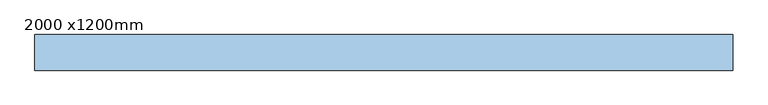
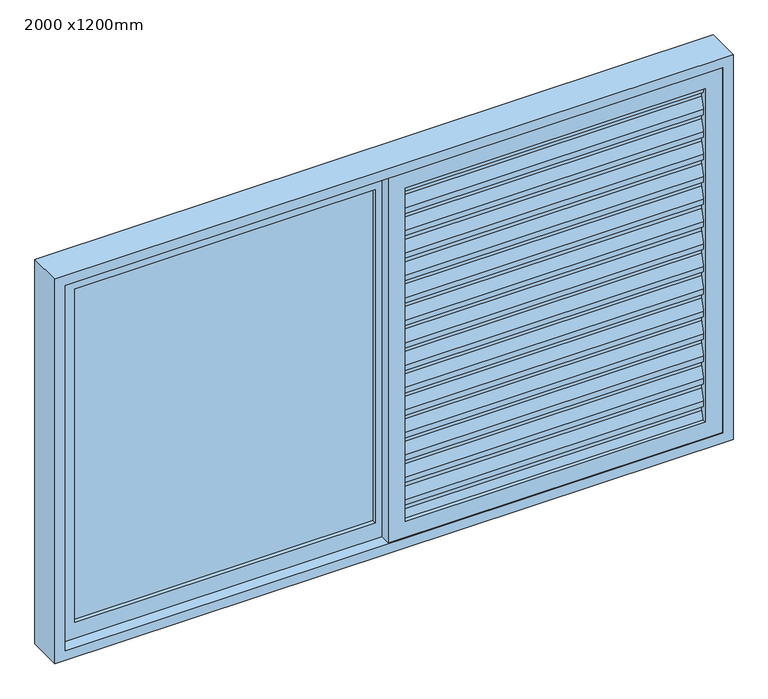
"""IFC4 building model written with IfcOpenShell, lengths in millimetres: window geometry, Janela Veneziana de Correr - 3 Folhas : 2000 x1200mm."""

import ifcopenshell
import ifcopenshell.guid

model = None  # the IFC model being written
_history = None  # IfcOwnerHistory: only IFC2X3 demands one
_inside = {}  # id of a spatial element -> (the spatial element, [elements in it])
_under = {}  # id of a project, library or spatial element -> (it, [spatial elements below it])
_declared = {}  # id of a project -> (the project, [libraries it declares])
_typed = {}  # id of a type object -> (the type object, [elements of that type])
_made_of = {}  # id of a material, layer set ... -> (it, [elements and type objects made of it])


def new_model(schema):
    """Start an empty IFC model of exactly this schema.

    Asked for "IFC4X3", IfcOpenShell would pick the latest addendum, in which some entities
    have other attributes; the version numbers below select the first issue.
    IFC2X3 requires an IfcOwnerHistory on every rooted entity: one is made here for all.
    """
    global model, _history
    if schema == "IFC4X3":
        model = ifcopenshell.file(schema_version=(4, 3, 0, 0))
    else:
        model = ifcopenshell.file(schema=schema)
    _inside.clear()
    _under.clear()
    _declared.clear()
    _typed.clear()
    _made_of.clear()
    _history = None
    if model.schema == "IFC2X3":
        org = make("IfcOrganization", Name="unknown")
        user = make(
            "IfcPersonAndOrganization",
            ThePerson=make("IfcPerson", FamilyName="unknown"),
            TheOrganization=org,
        )
        app = make(
            "IfcApplication",
            ApplicationDeveloper=org,
            Version="unknown",
            ApplicationFullName="unknown",
            ApplicationIdentifier="unknown",
        )
        _history = make(
            "IfcOwnerHistory",
            OwningUser=user,
            OwningApplication=app,
            ChangeAction="ADDED",
            CreationDate=0,
        )
    return model


def make(cls, **values):
    """One entity of the class cls with the attributes given. An attribute that is None is left unset."""
    return model.create_entity(
        cls, **{name: value for name, value in values.items() if value is not None}
    )


def rooted(cls, **values):
    """An entity with a GlobalId (a new one), such as an element, a storey or a relation."""
    return make(cls, GlobalId=ifcopenshell.guid.new(), OwnerHistory=_history, **values)


def si_unit(unit_type, name, prefix=None):
    """IfcSIUnit, for example si_unit("LENGTHUNIT", "METRE", prefix="MILLI")."""
    return make("IfcSIUnit", UnitType=unit_type, Prefix=prefix, Name=name)


def assignment(units):
    """IfcUnitAssignment: the units of a project."""
    return None if units is None else make("IfcUnitAssignment", Units=units)


def point(xyz):
    """IfcCartesianPoint."""
    return None if xyz is None else make("IfcCartesianPoint", Coordinates=xyz)


def direction(xyz):
    """IfcDirection."""
    return None if xyz is None else make("IfcDirection", DirectionRatios=xyz)


def frame(location, z_axis=None, x_axis=None):
    """IfcAxis2Placement3D, a coordinate frame: its origin and axes. An axis left out is left unset."""
    return make(
        "IfcAxis2Placement3D",
        Location=point(location),
        Axis=direction(z_axis),
        RefDirection=direction(x_axis),
    )


def origin():
    """The frame at (0, 0, 0) with its axes left unset."""
    return frame((0.0, 0.0, 0.0))


def place(relative_to, where):
    """IfcLocalPlacement: puts the frame where relative to a parent placement (None: the world)."""
    return make(
        "IfcLocalPlacement", PlacementRelTo=relative_to, RelativePlacement=where
    )


def context(
    kind, dimensions, precision=None, world=None, true_north=None, identifier=None
):
    """IfcGeometricRepresentationContext, for example the 3D "Model" context."""
    return make(
        "IfcGeometricRepresentationContext",
        ContextIdentifier=identifier,
        ContextType=kind,
        CoordinateSpaceDimension=dimensions,
        Precision=precision,
        WorldCoordinateSystem=world,
        TrueNorth=true_north,
    )


def project(units=None, contexts=None):
    """IfcProject with its units and contexts."""
    return rooted(
        "IfcProject",
        Name="project",
        RepresentationContexts=contexts,
        UnitsInContext=assignment(units),
    )


def spatial(cls, under=None, at=None, **own):
    """A site, building, storey or space (cls), placed at a placement, below another one or the project."""
    s = rooted(cls, ObjectPlacement=at, **own)
    if under is not None:
        _under.setdefault(under.id(), (under, []))[1].append(s)
    return s


def polyline(points):
    """IfcPolyline through the points."""
    return make("IfcPolyline", Points=[point(p) for p in points])


def outline(outer, holes=None, kind="AREA"):
    """IfcArbitraryClosedProfileDef: a profile drawn as a closed curve; with holes, ...WithVoids."""
    if holes is None:
        return make("IfcArbitraryClosedProfileDef", ProfileType=kind, OuterCurve=outer)
    return make(
        "IfcArbitraryProfileDefWithVoids",
        ProfileType=kind,
        OuterCurve=outer,
        InnerCurves=holes,
    )


def extrude(swept, where, along, depth):
    """IfcExtrudedAreaSolid: the profile swept, set in the frame where, extruded along a direction by depth."""
    return make(
        "IfcExtrudedAreaSolid",
        SweptArea=swept,
        Position=where,
        ExtrudedDirection=direction(along),
        Depth=depth,
    )


def shape(context_of_items, identifier, shape_type, items):
    """IfcShapeRepresentation: the items that make up one representation, for example the "Body"."""
    return make(
        "IfcShapeRepresentation",
        ContextOfItems=context_of_items,
        RepresentationIdentifier=identifier,
        RepresentationType=shape_type,
        Items=items,
    )


def source(mapping_origin, context_of_items, identifier, shape_type, items):
    """IfcRepresentationMap: a shape defined once, which mapped items show again and again."""
    return make(
        "IfcRepresentationMap",
        MappingOrigin=mapping_origin,
        MappedRepresentation=shape(context_of_items, identifier, shape_type, items),
    )


def transform(
    local_origin,
    x_axis=None,
    y_axis=None,
    z_axis=None,
    scale=None,
    scale2=None,
    scale3=None,
    uniform=True,
):
    """IfcCartesianTransformationOperator3D, or its non-uniform kind. x_axis, y_axis, z_axis: its Axis1, 2, 3."""
    if uniform:
        return make(
            "IfcCartesianTransformationOperator3D",
            Axis1=direction(x_axis),
            Axis2=direction(y_axis),
            LocalOrigin=point(local_origin),
            Scale=scale,
            Axis3=direction(z_axis),
        )
    return make(
        "IfcCartesianTransformationOperator3DnonUniform",
        Axis1=direction(x_axis),
        Axis2=direction(y_axis),
        LocalOrigin=point(local_origin),
        Scale=scale,
        Axis3=direction(z_axis),
        Scale2=scale2,
        Scale3=scale3,
    )


def mapped(mapping_source, mapping_target):
    """IfcMappedItem: shows the shape of a source again, moved by a transform."""
    return make(
        "IfcMappedItem", MappingSource=mapping_source, MappingTarget=mapping_target
    )


def made_of(thing, what):
    """Note that an element or type object is made of a material, layer set ...; save() writes the relation."""
    if what is not None:
        _made_of.setdefault(what.id(), (what, []))[1].append(thing)
    return thing


def element(
    cls,
    number,
    at=None,
    inside=None,
    cuts=None,
    type_object=None,
    material=None,
    context=None,
    identifier="Body",
    shape_type=None,
    held_by="IfcProductDefinitionShape",
    body=None,
    shapes=None,
    **own,
):
    """One element of the class cls, such as IfcWall. Its Tag is "e" and its number.

    at: its placement. inside: the storey or other place that contains it. cuts: it is an
    opening in that element (IfcRelVoidsElement). A single representation is given by context,
    identifier, shape_type and body (its items); several are given by shapes. held_by: the class
    of the entity that holds the representations. save() writes the other relations.
    """
    e = rooted(cls, Tag="e%d" % number, ObjectPlacement=at, **own)
    if body is not None:
        shapes = [shape(context, identifier, shape_type, body)]
    if shapes is not None:
        e.Representation = make(held_by, Representations=shapes)
    if inside is not None:
        _inside.setdefault(inside.id(), (inside, []))[1].append(e)
    if cuts is not None:
        rooted(
            "IfcRelVoidsElement", RelatingBuildingElement=cuts, RelatedOpeningElement=e
        )
    if type_object is not None:
        _typed.setdefault(type_object.id(), (type_object, []))[1].append(e)
    return made_of(e, material)


def aggregate(whole, parts):
    """IfcRelAggregates: a whole, such as a stair, and the parts it consists of."""
    return rooted("IfcRelAggregates", RelatingObject=whole, RelatedObjects=parts)


def save(model, path):
    """Write the relations noted so far, then the file.

    IfcRelAggregates (storeys below a building ...), IfcRelContainedInSpatialStructure (elements
    in a storey), IfcRelDefinesByType, IfcRelAssociatesMaterial and IfcRelDeclares: one each for
    every whole, place, type object, material and project.
    """
    for whole, parts in _under.values():
        aggregate(whole, parts)
    for where, things in _inside.values():
        rooted(
            "IfcRelContainedInSpatialStructure",
            RelatedElements=things,
            RelatingStructure=where,
        )
    for kind, things in _typed.values():
        rooted("IfcRelDefinesByType", RelatedObjects=things, RelatingType=kind)
    for what, things in _made_of.values():
        rooted("IfcRelAssociatesMaterial", RelatedObjects=things, RelatingMaterial=what)
    for by, libraries in _declared.values():
        rooted("IfcRelDeclares", RelatingContext=by, RelatedDefinitions=libraries)
    model.write(path)


def window_2000_x1200mm_dbfbffcb(model_context):
    return source(origin(), model_context, "Body", "SweptSolid", [
        extrude(outline(polyline([(0.6, 1125.0), (0.6, 1105.0), (-6.5028414, 1080.1400549), (-7.5428571, 1080.1400549), (-0.4, 1105.1400549), (-0.4, 1124.0), (-10.4, 1124.0), (-10.4, 1140.1400549), (-0.4, 1175.1400549), (-0.4, 1194.0), (-10.4, 1194.0), (-10.4, 1210.1400549), (-0.4, 1245.1400549), (-0.4, 1264.0), (-10.4, 1264.0), (-10.4, 1280.1400549), (-0.4, 1315.1400549), (-0.4, 1334.0), (-10.4, 1334.0), (-10.4, 1350.1400549), (-0.4, 1385.1400549), (-0.4, 1404.0), (-10.4, 1404.0), (-10.4, 1420.1400549), (-0.4, 1455.1400549), (-0.4, 1474.0), (-10.4, 1474.0), (-10.4, 1490.1400549), (-0.4, 1525.1400549), (-0.4, 1544.0), (-10.4, 1544.0), (-10.4, 1560.1400549), (-0.4, 1595.1400549), (-0.4, 1614.0), (-10.4, 1614.0), (-10.4, 1630.1400549), (-0.4, 1665.1400549), (-0.4, 1684.0), (-10.4, 1684.0), (-10.4, 1700.1400549), (-0.4, 1735.1400549), (-0.4, 1754.0), (-10.4, 1754.0), (-10.4, 1770.1400549), (-0.4, 1805.1400549), (-0.4, 1824.0), (-10.4, 1824.0), (-10.4, 1840.1400549), (-0.4, 1875.1400549), (-0.4, 1894.0), (-10.4, 1894.0), (-10.4, 1910.1400549), (-0.4, 1945.1400549), (-0.4, 1964.0), (-10.4, 1964.0), (-10.4, 1980.1400549), (-0.4, 2015.1400549), (-0.4, 2034.0), (-10.4, 2034.0), (-10.4, 2050.1400549), (-0.4, 2085.1400549), (-0.4, 2104.0), (-10.4, 2104.0), (-10.4, 2120.1400549), (-9.4, 2120.0), (-9.4, 2105.0), (0.6, 2105.0), (0.6, 2085.0), (-9.4, 2050.0), (-9.4, 2035.0), (0.6, 2035.0), (0.6, 2015.0), (-9.4, 1980.0), (-9.4, 1965.0), (0.6, 1965.0), (0.6, 1945.0), (-9.4, 1910.0), (-9.4, 1895.0), (0.6, 1895.0), (0.6, 1875.0), (-9.4, 1840.0), (-9.4, 1825.0), (0.6, 1825.0), (0.6, 1805.0), (-9.4, 1770.0), (-9.4, 1755.0), (0.6, 1755.0), (0.6, 1735.0), (-9.4, 1700.0), (-9.4, 1685.0), (0.6, 1685.0), (0.6, 1665.0), (-9.4, 1630.0), (-9.4, 1615.0), (0.6, 1615.0), (0.6, 1595.0), (-9.4, 1560.0), (-9.4, 1545.0), (0.6, 1545.0), (0.6, 1525.0), (-9.4, 1490.0), (-9.4, 1475.0), (0.6, 1475.0), (0.6, 1455.0), (-9.4, 1420.0), (-9.4, 1405.0), (0.6, 1405.0), (0.6, 1385.0), (-9.4, 1350.0), (-9.4, 1335.0), (0.6, 1335.0), (0.6, 1315.0), (-9.4, 1280.0), (-9.4, 1265.0), (0.6, 1265.0), (0.6, 1245.0), (-9.4, 1210.0), (-9.4, 1195.0), (0.6, 1195.0), (0.6, 1175.0), (-9.4, 1140.0), (-9.4, 1125.0), (0.6, 1125.0)])), frame((35.0, 0.0, 0.0), z_axis=(1.0, 0.0, 0.0), x_axis=(0.0, 1.0, 0.0)), (0.0, 0.0, 1.0), 965.0),
        extrude(outline(polyline([(66.6, 1125.0), (66.6, 1105.0), (59.4971586, 1080.1400549), (58.4571429, 1080.1400549), (65.6, 1105.1400549), (65.6, 1124.0), (55.6, 1124.0), (55.6, 1140.1400549), (65.6, 1175.1400549), (65.6, 1194.0), (55.6, 1194.0), (55.6, 1210.1400549), (65.6, 1245.1400549), (65.6, 1264.0), (55.6, 1264.0), (55.6, 1280.1400549), (65.6, 1315.1400549), (65.6, 1334.0), (55.6, 1334.0), (55.6, 1350.1400549), (65.6, 1385.1400549), (65.6, 1404.0), (55.6, 1404.0), (55.6, 1420.1400549), (65.6, 1455.1400549), (65.6, 1474.0), (55.6, 1474.0), (55.6, 1490.1400549), (65.6, 1525.1400549), (65.6, 1544.0), (55.6, 1544.0), (55.6, 1560.1400549), (65.6, 1595.1400549), (65.6, 1614.0), (55.6, 1614.0), (55.6, 1630.1400549), (65.6, 1665.1400549), (65.6, 1684.0), (55.6, 1684.0), (55.6, 1700.1400549), (65.6, 1735.1400549), (65.6, 1754.0), (55.6, 1754.0), (55.6, 1770.1400549), (65.6, 1805.1400549), (65.6, 1824.0), (55.6, 1824.0), (55.6, 1840.1400549), (65.6, 1875.1400549), (65.6, 1894.0), (55.6, 1894.0), (55.6, 1910.1400549), (65.6, 1945.1400549), (65.6, 1964.0), (55.6, 1964.0), (55.6, 1980.1400549), (65.6, 2015.1400549), (65.6, 2034.0), (55.6, 2034.0), (55.6, 2050.1400549), (65.6, 2085.1400549), (65.6, 2104.0), (55.6, 2104.0), (55.6, 2120.1400549), (56.6, 2120.0), (56.6, 2105.0), (66.6, 2105.0), (66.6, 2085.0), (56.6, 2050.0), (56.6, 2035.0), (66.6, 2035.0), (66.6, 2015.0), (56.6, 1980.0), (56.6, 1965.0), (66.6, 1965.0), (66.6, 1945.0), (56.6, 1910.0), (56.6, 1895.0), (66.6, 1895.0), (66.6, 1875.0), (56.6, 1840.0), (56.6, 1825.0), (66.6, 1825.0), (66.6, 1805.0), (56.6, 1770.0), (56.6, 1755.0), (66.6, 1755.0), (66.6, 1735.0), (56.6, 1700.0), (56.6, 1685.0), (66.6, 1685.0), (66.6, 1665.0), (56.6, 1630.0), (56.6, 1615.0), (66.6, 1615.0), (66.6, 1595.0), (56.6, 1560.0), (56.6, 1545.0), (66.6, 1545.0), (66.6, 1525.0), (56.6, 1490.0), (56.6, 1475.0), (66.6, 1475.0), (66.6, 1455.0), (56.6, 1420.0), (56.6, 1405.0), (66.6, 1405.0), (66.6, 1385.0), (56.6, 1350.0), (56.6, 1335.0), (66.6, 1335.0), (66.6, 1315.0), (56.6, 1280.0), (56.6, 1265.0), (66.6, 1265.0), (66.6, 1245.0), (56.6, 1210.0), (56.6, 1195.0), (66.6, 1195.0), (66.6, 1175.0), (56.6, 1140.0), (56.6, 1125.0), (66.6, 1125.0)])), frame((35.0, 0.0, 0.0), z_axis=(1.0, 0.0, 0.0), x_axis=(0.0, 1.0, 0.0)), (0.0, 0.0, 1.0), 965.0),
        extrude(outline(polyline([(2170.0, -15.0), (1030.0, -15.0), (1030.0, 970.0), (2170.0, 970.0), (2170.0, -15.0)]), holes=[polyline([(2120.0, 35.0), (2120.0, 920.0), (1080.0, 920.0), (1080.0, 35.0), (2120.0, 35.0)])]), frame((0.0, -19.4, 0.0), z_axis=(0.0, 1.0, 0.0), x_axis=(0.0, 0.0, 1.0)), (0.0, 0.0, 1.0), 30.0),
        extrude(outline(polyline([(2170.0, -15.0), (1030.0, -15.0), (1030.0, 970.0), (2170.0, 970.0), (2170.0, -15.0)]), holes=[polyline([(2120.0, 35.0), (2120.0, 920.0), (1080.0, 920.0), (1080.0, 35.0), (2120.0, 35.0)])]), frame((0.0, 46.6, 0.0), z_axis=(0.0, 1.0, 0.0), x_axis=(0.0, 0.0, 1.0)), (0.0, 0.0, 1.0), 30.0),
        extrude(outline(polyline([(-920.0, 25.1), (-920.0, 32.1), (-35.0, 32.1), (-35.0, 25.1), (-920.0, 25.1)])), frame((0.0, 0.0, 1080.0), z_axis=(0.0, 0.0, 1.0), x_axis=(1.0, 0.0, 0.0)), (0.0, 0.0, 1.0), 1040.0),
        extrude(outline(polyline([(2170.0, 15.0), (2170.0, -970.0), (1030.0, -970.0), (1030.0, 15.0), (2170.0, 15.0)]), holes=[polyline([(2120.0, -35.0), (1080.0, -35.0), (1080.0, -920.0), (2120.0, -920.0), (2120.0, -35.0)])]), frame((0.0, 13.6, 0.0), z_axis=(0.0, 1.0, 0.0), x_axis=(0.0, 0.0, 1.0)), (0.0, 0.0, 1.0), 30.0),
        extrude(outline(polyline([(2200.0, 1000.0), (2200.0, -1000.0), (1000.0, -1000.0), (1000.0, 1000.0), (2200.0, 1000.0)]), holes=[polyline([(2170.0, 970.0), (1030.0, 970.0), (1030.0, -970.0), (2170.0, -970.0), (2170.0, 970.0)])]), frame((0.0, -22.4, 0.0), z_axis=(0.0, 1.0, 0.0), x_axis=(0.0, 0.0, 1.0)), (0.0, 0.0, 1.0), 102.0),
    ])


if __name__ == "__main__":
    model = new_model("IFC4")
    model_context = context("Model", 3, world=origin())
    ifc_project = project(units=[si_unit("LENGTHUNIT", "METRE", prefix="MILLI")], contexts=[model_context])
    site = spatial("IfcSite", under=ifc_project)
    building = spatial("IfcBuilding", under=site)
    placement = place(None, origin())
    window_2000_x1200mm_shape = window_2000_x1200mm_dbfbffcb(model_context)
    element("IfcWindow", 1, ObjectType="Janela Veneziana de Correr - 3 Folhas : 2000 x1200mm", at=placement, inside=building, context=model_context, shape_type="MappedRepresentation", body=[
        mapped(window_2000_x1200mm_shape, transform((0.0, 0.0, 0.0), x_axis=(1.0, 0.0, 0.0), y_axis=(0.0, 1.0, 0.0), z_axis=(0.0, 0.0, 1.0))),
    ])
    save(model, "model.ifc")

# Revit data of these elements
# Type "Janela Veneziana de Correr - 3 Folhas : 2000 x1200mm"
#   Type Mark = "J13"
#   SINAPI = ""
#   Tolerância = 0.003 m
#   Módulo Básico M = 0.10 m
#   Largura de Coordenação Modular CM = 2.00 m
#   Largura Vão = 0.965 m
#   Largura Veneziana = 1.00 m
#   Espessura Montante = 0.03 m
#   Largura Batente = 0.10 m
#   L_est_v marco = 0.05 m
#   L_est_h_marco = 0.05 m
#   L_contramarco = 0.03 m
#   Altura de Coordenação Modular CM = 1.20 m
#   Altura Peitoril = 0.95 m
#   Height = 1.20 m
#   Width = 2.00 m
#   Número de Módulos Básicos nM Largura = 20
#   Número de Módulos Básicos nM Altura = 12
#   Material estrutura = Metal - Alumínio
#   Material Quadro = Metal - Alumínio
#   Material Painel = Vidro
#   Type Comments = ""
#   Wall Closure = (empty or 0)
#   Construction Type = (empty or 0)
#   Assembly Code = ""
# Element 1 (IfcWindow, "Janela Veneziana de Correr - 3 Folhas : 2000 x1200mm")
#   Materials on its faces: "Metal - Alumínio", "Vidro"
# Materials
#   "Metal - Alumínio": class "Metal", colour RGB 244 244 244, transparency 0
#   "Vidro": class "Vidro", colour RGB 0 128 192, transparency 0.9, Description = "Vidro de sílica", Cost = 0
